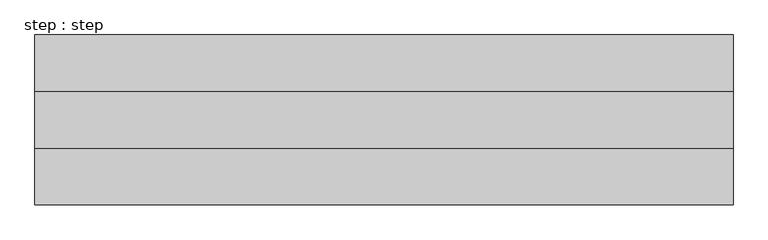
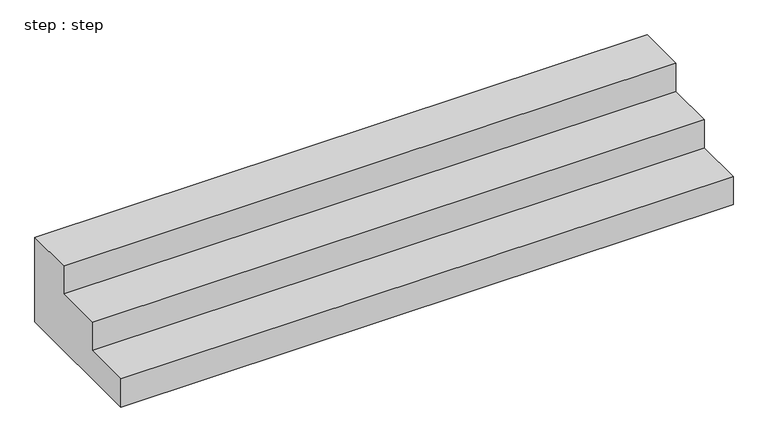
"""IFC4 building model written with IfcOpenShell, lengths in millimetres: proxy geometry, step : step."""

import ifcopenshell
import ifcopenshell.guid

model = None  # the IFC model being written
_history = None  # IfcOwnerHistory: only IFC2X3 demands one
_inside = {}  # id of a spatial element -> (the spatial element, [elements in it])
_under = {}  # id of a project, library or spatial element -> (it, [spatial elements below it])
_declared = {}  # id of a project -> (the project, [libraries it declares])
_typed = {}  # id of a type object -> (the type object, [elements of that type])
_made_of = {}  # id of a material, layer set ... -> (it, [elements and type objects made of it])


def new_model(schema):
    """Start an empty IFC model of exactly this schema.

    Asked for "IFC4X3", IfcOpenShell would pick the latest addendum, in which some entities
    have other attributes; the version numbers below select the first issue.
    IFC2X3 requires an IfcOwnerHistory on every rooted entity: one is made here for all.
    """
    global model, _history
    if schema == "IFC4X3":
        model = ifcopenshell.file(schema_version=(4, 3, 0, 0))
    else:
        model = ifcopenshell.file(schema=schema)
    _inside.clear()
    _under.clear()
    _declared.clear()
    _typed.clear()
    _made_of.clear()
    _history = None
    if model.schema == "IFC2X3":
        org = make("IfcOrganization", Name="unknown")
        user = make(
            "IfcPersonAndOrganization",
            ThePerson=make("IfcPerson", FamilyName="unknown"),
            TheOrganization=org,
        )
        app = make(
            "IfcApplication",
            ApplicationDeveloper=org,
            Version="unknown",
            ApplicationFullName="unknown",
            ApplicationIdentifier="unknown",
        )
        _history = make(
            "IfcOwnerHistory",
            OwningUser=user,
            OwningApplication=app,
            ChangeAction="ADDED",
            CreationDate=0,
        )
    return model


def make(cls, **values):
    """One entity of the class cls with the attributes given. An attribute that is None is left unset."""
    return model.create_entity(
        cls, **{name: value for name, value in values.items() if value is not None}
    )


def rooted(cls, **values):
    """An entity with a GlobalId (a new one), such as an element, a storey or a relation."""
    return make(cls, GlobalId=ifcopenshell.guid.new(), OwnerHistory=_history, **values)


def si_unit(unit_type, name, prefix=None):
    """IfcSIUnit, for example si_unit("LENGTHUNIT", "METRE", prefix="MILLI")."""
    return make("IfcSIUnit", UnitType=unit_type, Prefix=prefix, Name=name)


def assignment(units):
    """IfcUnitAssignment: the units of a project."""
    return None if units is None else make("IfcUnitAssignment", Units=units)


def point(xyz):
    """IfcCartesianPoint."""
    return None if xyz is None else make("IfcCartesianPoint", Coordinates=xyz)


def direction(xyz):
    """IfcDirection."""
    return None if xyz is None else make("IfcDirection", DirectionRatios=xyz)


def frame(location, z_axis=None, x_axis=None):
    """IfcAxis2Placement3D, a coordinate frame: its origin and axes. An axis left out is left unset."""
    return make(
        "IfcAxis2Placement3D",
        Location=point(location),
        Axis=direction(z_axis),
        RefDirection=direction(x_axis),
    )


def origin():
    """The frame at (0, 0, 0) with its axes left unset."""
    return frame((0.0, 0.0, 0.0))


def place(relative_to, where):
    """IfcLocalPlacement: puts the frame where relative to a parent placement (None: the world)."""
    return make(
        "IfcLocalPlacement", PlacementRelTo=relative_to, RelativePlacement=where
    )


def context(
    kind, dimensions, precision=None, world=None, true_north=None, identifier=None
):
    """IfcGeometricRepresentationContext, for example the 3D "Model" context."""
    return make(
        "IfcGeometricRepresentationContext",
        ContextIdentifier=identifier,
        ContextType=kind,
        CoordinateSpaceDimension=dimensions,
        Precision=precision,
        WorldCoordinateSystem=world,
        TrueNorth=true_north,
    )


def project(units=None, contexts=None):
    """IfcProject with its units and contexts."""
    return rooted(
        "IfcProject",
        Name="project",
        RepresentationContexts=contexts,
        UnitsInContext=assignment(units),
    )


def spatial(cls, under=None, at=None, **own):
    """A site, building, storey or space (cls), placed at a placement, below another one or the project."""
    s = rooted(cls, ObjectPlacement=at, **own)
    if under is not None:
        _under.setdefault(under.id(), (under, []))[1].append(s)
    return s


def polyline(points):
    """IfcPolyline through the points."""
    return make("IfcPolyline", Points=[point(p) for p in points])


def outline(outer, holes=None, kind="AREA"):
    """IfcArbitraryClosedProfileDef: a profile drawn as a closed curve; with holes, ...WithVoids."""
    if holes is None:
        return make("IfcArbitraryClosedProfileDef", ProfileType=kind, OuterCurve=outer)
    return make(
        "IfcArbitraryProfileDefWithVoids",
        ProfileType=kind,
        OuterCurve=outer,
        InnerCurves=holes,
    )


def extrude(swept, where, along, depth):
    """IfcExtrudedAreaSolid: the profile swept, set in the frame where, extruded along a direction by depth."""
    return make(
        "IfcExtrudedAreaSolid",
        SweptArea=swept,
        Position=where,
        ExtrudedDirection=direction(along),
        Depth=depth,
    )


def shape(context_of_items, identifier, shape_type, items):
    """IfcShapeRepresentation: the items that make up one representation, for example the "Body"."""
    return make(
        "IfcShapeRepresentation",
        ContextOfItems=context_of_items,
        RepresentationIdentifier=identifier,
        RepresentationType=shape_type,
        Items=items,
    )


def source(mapping_origin, context_of_items, identifier, shape_type, items):
    """IfcRepresentationMap: a shape defined once, which mapped items show again and again."""
    return make(
        "IfcRepresentationMap",
        MappingOrigin=mapping_origin,
        MappedRepresentation=shape(context_of_items, identifier, shape_type, items),
    )


def transform(
    local_origin,
    x_axis=None,
    y_axis=None,
    z_axis=None,
    scale=None,
    scale2=None,
    scale3=None,
    uniform=True,
):
    """IfcCartesianTransformationOperator3D, or its non-uniform kind. x_axis, y_axis, z_axis: its Axis1, 2, 3."""
    if uniform:
        return make(
            "IfcCartesianTransformationOperator3D",
            Axis1=direction(x_axis),
            Axis2=direction(y_axis),
            LocalOrigin=point(local_origin),
            Scale=scale,
            Axis3=direction(z_axis),
        )
    return make(
        "IfcCartesianTransformationOperator3DnonUniform",
        Axis1=direction(x_axis),
        Axis2=direction(y_axis),
        LocalOrigin=point(local_origin),
        Scale=scale,
        Axis3=direction(z_axis),
        Scale2=scale2,
        Scale3=scale3,
    )


def mapped(mapping_source, mapping_target):
    """IfcMappedItem: shows the shape of a source again, moved by a transform."""
    return make(
        "IfcMappedItem", MappingSource=mapping_source, MappingTarget=mapping_target
    )


def made_of(thing, what):
    """Note that an element or type object is made of a material, layer set ...; save() writes the relation."""
    if what is not None:
        _made_of.setdefault(what.id(), (what, []))[1].append(thing)
    return thing


def element(
    cls,
    number,
    at=None,
    inside=None,
    cuts=None,
    type_object=None,
    material=None,
    context=None,
    identifier="Body",
    shape_type=None,
    held_by="IfcProductDefinitionShape",
    body=None,
    shapes=None,
    **own,
):
    """One element of the class cls, such as IfcWall. Its Tag is "e" and its number.

    at: its placement. inside: the storey or other place that contains it. cuts: it is an
    opening in that element (IfcRelVoidsElement). A single representation is given by context,
    identifier, shape_type and body (its items); several are given by shapes. held_by: the class
    of the entity that holds the representations. save() writes the other relations.
    """
    e = rooted(cls, Tag="e%d" % number, ObjectPlacement=at, **own)
    if body is not None:
        shapes = [shape(context, identifier, shape_type, body)]
    if shapes is not None:
        e.Representation = make(held_by, Representations=shapes)
    if inside is not None:
        _inside.setdefault(inside.id(), (inside, []))[1].append(e)
    if cuts is not None:
        rooted(
            "IfcRelVoidsElement", RelatingBuildingElement=cuts, RelatedOpeningElement=e
        )
    if type_object is not None:
        _typed.setdefault(type_object.id(), (type_object, []))[1].append(e)
    return made_of(e, material)


def aggregate(whole, parts):
    """IfcRelAggregates: a whole, such as a stair, and the parts it consists of."""
    return rooted("IfcRelAggregates", RelatingObject=whole, RelatedObjects=parts)


def save(model, path):
    """Write the relations noted so far, then the file.

    IfcRelAggregates (storeys below a building ...), IfcRelContainedInSpatialStructure (elements
    in a storey), IfcRelDefinesByType, IfcRelAssociatesMaterial and IfcRelDeclares: one each for
    every whole, place, type object, material and project.
    """
    for whole, parts in _under.values():
        aggregate(whole, parts)
    for where, things in _inside.values():
        rooted(
            "IfcRelContainedInSpatialStructure",
            RelatedElements=things,
            RelatingStructure=where,
        )
    for kind, things in _typed.values():
        rooted("IfcRelDefinesByType", RelatedObjects=things, RelatingType=kind)
    for what, things in _made_of.values():
        rooted("IfcRelAssociatesMaterial", RelatedObjects=things, RelatingMaterial=what)
    for by, libraries in _declared.values():
        rooted("IfcRelDeclares", RelatingContext=by, RelatedDefinitions=libraries)
    model.write(path)


def step_step_1a2821ed(model_context):
    return source(origin(), model_context, "Body", "SweptSolid", [
        extrude(outline(polyline([(-3204.9933886, 450.0), (-2954.9933886, 450.0), (-2954.9933886, 0.0), (-3704.9933886, 0.0), (-3704.9933886, 150.0), (-3454.9933886, 150.0), (-3454.9933886, 300.0), (-3204.9933886, 300.0), (-3204.9933886, 450.0)])), frame((-15676.5903863, 0.0, 0.0), z_axis=(1.0, 0.0, 0.0), x_axis=(0.0, 1.0, 0.0)), (0.0, 0.0, 1.0), 3085.0),
    ])


if __name__ == "__main__":
    model = new_model("IFC4")
    model_context = context("Model", 3, world=origin())
    ifc_project = project(units=[si_unit("LENGTHUNIT", "METRE", prefix="MILLI")], contexts=[model_context])
    site = spatial("IfcSite", under=ifc_project)
    building = spatial("IfcBuilding", under=site)
    placement = place(None, origin())
    step_step_shape = step_step_1a2821ed(model_context)
    element("IfcBuildingElementProxy", 1, Name="step : step", ObjectType="step : step", at=placement, inside=building, context=model_context, shape_type="MappedRepresentation", body=[
        mapped(step_step_shape, transform((0.0, 0.0, 0.0), x_axis=(1.0, 0.0, 0.0), y_axis=(0.0, 1.0, 0.0), z_axis=(0.0, 0.0, 1.0))),
    ])
    save(model, "model.ifc")

# Revit data of these elements
# Project information
#   Project Issue Date = "Issue Date"
#   Project Status = "Project Status"
#   Client Name = "Owner"
#   Project Address = "Enter address here"
#   Project Name = "Project Name"
#   Project Number = "0001"
